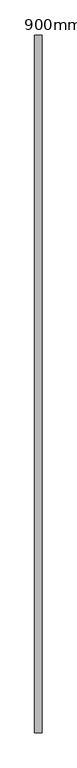
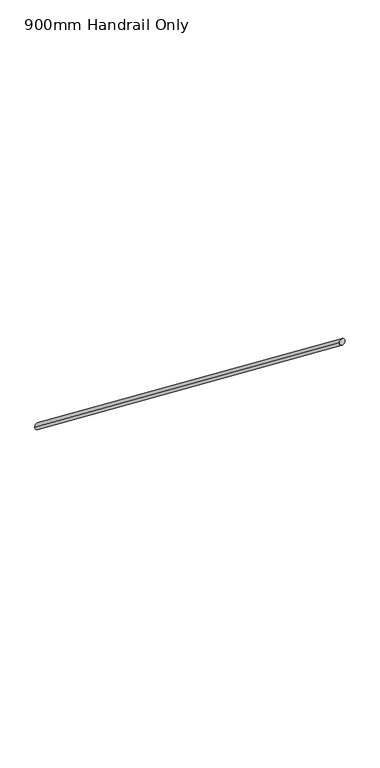
"""IFC4 building model written with IfcOpenShell, lengths in millimetres: railing geometry, 900mm Handrail Only."""

import ifcopenshell
import ifcopenshell.guid

model = None  # the IFC model being written
_history = None  # IfcOwnerHistory: only IFC2X3 demands one
_inside = {}  # id of a spatial element -> (the spatial element, [elements in it])
_under = {}  # id of a project, library or spatial element -> (it, [spatial elements below it])
_declared = {}  # id of a project -> (the project, [libraries it declares])
_typed = {}  # id of a type object -> (the type object, [elements of that type])
_made_of = {}  # id of a material, layer set ... -> (it, [elements and type objects made of it])


def new_model(schema):
    """Start an empty IFC model of exactly this schema.

    Asked for "IFC4X3", IfcOpenShell would pick the latest addendum, in which some entities
    have other attributes; the version numbers below select the first issue.
    IFC2X3 requires an IfcOwnerHistory on every rooted entity: one is made here for all.
    """
    global model, _history
    if schema == "IFC4X3":
        model = ifcopenshell.file(schema_version=(4, 3, 0, 0))
    else:
        model = ifcopenshell.file(schema=schema)
    _inside.clear()
    _under.clear()
    _declared.clear()
    _typed.clear()
    _made_of.clear()
    _history = None
    if model.schema == "IFC2X3":
        org = make("IfcOrganization", Name="unknown")
        user = make(
            "IfcPersonAndOrganization",
            ThePerson=make("IfcPerson", FamilyName="unknown"),
            TheOrganization=org,
        )
        app = make(
            "IfcApplication",
            ApplicationDeveloper=org,
            Version="unknown",
            ApplicationFullName="unknown",
            ApplicationIdentifier="unknown",
        )
        _history = make(
            "IfcOwnerHistory",
            OwningUser=user,
            OwningApplication=app,
            ChangeAction="ADDED",
            CreationDate=0,
        )
    return model


def make(cls, **values):
    """One entity of the class cls with the attributes given. An attribute that is None is left unset."""
    return model.create_entity(
        cls, **{name: value for name, value in values.items() if value is not None}
    )


def rooted(cls, **values):
    """An entity with a GlobalId (a new one), such as an element, a storey or a relation."""
    return make(cls, GlobalId=ifcopenshell.guid.new(), OwnerHistory=_history, **values)


def si_unit(unit_type, name, prefix=None):
    """IfcSIUnit, for example si_unit("LENGTHUNIT", "METRE", prefix="MILLI")."""
    return make("IfcSIUnit", UnitType=unit_type, Prefix=prefix, Name=name)


def assignment(units):
    """IfcUnitAssignment: the units of a project."""
    return None if units is None else make("IfcUnitAssignment", Units=units)


def point(xyz):
    """IfcCartesianPoint."""
    return None if xyz is None else make("IfcCartesianPoint", Coordinates=xyz)


def direction(xyz):
    """IfcDirection."""
    return None if xyz is None else make("IfcDirection", DirectionRatios=xyz)


def frame(location, z_axis=None, x_axis=None):
    """IfcAxis2Placement3D, a coordinate frame: its origin and axes. An axis left out is left unset."""
    return make(
        "IfcAxis2Placement3D",
        Location=point(location),
        Axis=direction(z_axis),
        RefDirection=direction(x_axis),
    )


def origin():
    """The frame at (0, 0, 0) with its axes left unset."""
    return frame((0.0, 0.0, 0.0))


def place(relative_to, where):
    """IfcLocalPlacement: puts the frame where relative to a parent placement (None: the world)."""
    return make(
        "IfcLocalPlacement", PlacementRelTo=relative_to, RelativePlacement=where
    )


def context(
    kind, dimensions, precision=None, world=None, true_north=None, identifier=None
):
    """IfcGeometricRepresentationContext, for example the 3D "Model" context."""
    return make(
        "IfcGeometricRepresentationContext",
        ContextIdentifier=identifier,
        ContextType=kind,
        CoordinateSpaceDimension=dimensions,
        Precision=precision,
        WorldCoordinateSystem=world,
        TrueNorth=true_north,
    )


def project(units=None, contexts=None):
    """IfcProject with its units and contexts."""
    return rooted(
        "IfcProject",
        Name="project",
        RepresentationContexts=contexts,
        UnitsInContext=assignment(units),
    )


def spatial(cls, under=None, at=None, **own):
    """A site, building, storey or space (cls), placed at a placement, below another one or the project."""
    s = rooted(cls, ObjectPlacement=at, **own)
    if under is not None:
        _under.setdefault(under.id(), (under, []))[1].append(s)
    return s


def ellipse_curve(where, semi_axis1, semi_axis2):
    """IfcEllipse in the frame where."""
    return make(
        "IfcEllipse", Position=where, SemiAxis1=semi_axis1, SemiAxis2=semi_axis2
    )


def shape(context_of_items, identifier, shape_type, items):
    """IfcShapeRepresentation: the items that make up one representation, for example the "Body"."""
    return make(
        "IfcShapeRepresentation",
        ContextOfItems=context_of_items,
        RepresentationIdentifier=identifier,
        RepresentationType=shape_type,
        Items=items,
    )


def source(mapping_origin, context_of_items, identifier, shape_type, items):
    """IfcRepresentationMap: a shape defined once, which mapped items show again and again."""
    return make(
        "IfcRepresentationMap",
        MappingOrigin=mapping_origin,
        MappedRepresentation=shape(context_of_items, identifier, shape_type, items),
    )


def transform(
    local_origin,
    x_axis=None,
    y_axis=None,
    z_axis=None,
    scale=None,
    scale2=None,
    scale3=None,
    uniform=True,
):
    """IfcCartesianTransformationOperator3D, or its non-uniform kind. x_axis, y_axis, z_axis: its Axis1, 2, 3."""
    if uniform:
        return make(
            "IfcCartesianTransformationOperator3D",
            Axis1=direction(x_axis),
            Axis2=direction(y_axis),
            LocalOrigin=point(local_origin),
            Scale=scale,
            Axis3=direction(z_axis),
        )
    return make(
        "IfcCartesianTransformationOperator3DnonUniform",
        Axis1=direction(x_axis),
        Axis2=direction(y_axis),
        LocalOrigin=point(local_origin),
        Scale=scale,
        Axis3=direction(z_axis),
        Scale2=scale2,
        Scale3=scale3,
    )


def mapped(mapping_source, mapping_target):
    """IfcMappedItem: shows the shape of a source again, moved by a transform."""
    return make(
        "IfcMappedItem", MappingSource=mapping_source, MappingTarget=mapping_target
    )


def made_of(thing, what):
    """Note that an element or type object is made of a material, layer set ...; save() writes the relation."""
    if what is not None:
        _made_of.setdefault(what.id(), (what, []))[1].append(thing)
    return thing


def element(
    cls,
    number,
    at=None,
    inside=None,
    cuts=None,
    type_object=None,
    material=None,
    context=None,
    identifier="Body",
    shape_type=None,
    held_by="IfcProductDefinitionShape",
    body=None,
    shapes=None,
    **own,
):
    """One element of the class cls, such as IfcWall. Its Tag is "e" and its number.

    at: its placement. inside: the storey or other place that contains it. cuts: it is an
    opening in that element (IfcRelVoidsElement). A single representation is given by context,
    identifier, shape_type and body (its items); several are given by shapes. held_by: the class
    of the entity that holds the representations. save() writes the other relations.
    """
    e = rooted(cls, Tag="e%d" % number, ObjectPlacement=at, **own)
    if body is not None:
        shapes = [shape(context, identifier, shape_type, body)]
    if shapes is not None:
        e.Representation = make(held_by, Representations=shapes)
    if inside is not None:
        _inside.setdefault(inside.id(), (inside, []))[1].append(e)
    if cuts is not None:
        rooted(
            "IfcRelVoidsElement", RelatingBuildingElement=cuts, RelatedOpeningElement=e
        )
    if type_object is not None:
        _typed.setdefault(type_object.id(), (type_object, []))[1].append(e)
    return made_of(e, material)


def aggregate(whole, parts):
    """IfcRelAggregates: a whole, such as a stair, and the parts it consists of."""
    return rooted("IfcRelAggregates", RelatingObject=whole, RelatedObjects=parts)


def save(model, path):
    """Write the relations noted so far, then the file.

    IfcRelAggregates (storeys below a building ...), IfcRelContainedInSpatialStructure (elements
    in a storey), IfcRelDefinesByType, IfcRelAssociatesMaterial and IfcRelDeclares: one each for
    every whole, place, type object, material and project.
    """
    for whole, parts in _under.values():
        aggregate(whole, parts)
    for where, things in _inside.values():
        rooted(
            "IfcRelContainedInSpatialStructure",
            RelatedElements=things,
            RelatingStructure=where,
        )
    for kind, things in _typed.values():
        rooted("IfcRelDefinesByType", RelatedObjects=things, RelatingType=kind)
    for what, things in _made_of.values():
        rooted("IfcRelAssociatesMaterial", RelatedObjects=things, RelatingMaterial=what)
    for by, libraries in _declared.values():
        rooted("IfcRelDeclares", RelatingContext=by, RelatedDefinitions=libraries)
    model.write(path)


def plane_surface(at):
    """IfcPlane: the flat surface through the origin of the frame at, square to its z axis."""
    return make("IfcPlane", Position=at)


def cylinder_surface(at, radius):
    """IfcCylindricalSurface: all points at the distance radius from the z axis of the frame at."""
    return make("IfcCylindricalSurface", Position=at, Radius=radius)


def advanced_brep(points, edges, surfaces, faces):
    """IfcAdvancedBrep: a solid bounded by faces that lie on surfaces and meet in shared edges.

    An edge is (start, end): straight between two places in points (the first is 0);
    or (start, end, curve); or (start, end, curve, False) where it runs against its curve.
    A face is (place in surfaces, loops), or (place, loops, False) where it looks against
    its surface's normal. A loop lists edges by number (the first is 1), with a minus sign
    where the edge is run from its end to its start. The first loop is the outer one.
    """
    corners = [point(p) for p in points]
    vertices = [make("IfcVertexPoint", VertexGeometry=c) for c in corners]
    made = []
    for start, end, *more in edges:
        made.append(
            make(
                "IfcEdgeCurve",
                EdgeStart=vertices[start],
                EdgeEnd=vertices[end],
                EdgeGeometry=more[0] if more else make("IfcPolyline", Points=[corners[start], corners[end]]),
                SameSense=more[1] if len(more) > 1 else True,
            )
        )
    hull = []
    for where, loops, *sense in faces:
        bounds = []
        for j, loop in enumerate(loops):
            ring = [make("IfcOrientedEdge", EdgeElement=made[abs(k) - 1], Orientation=k > 0) for k in loop]
            bounds.append(
                make(
                    "IfcFaceOuterBound" if j == 0 else "IfcFaceBound",
                    Bound=make("IfcEdgeLoop", EdgeList=ring),
                    Orientation=True,
                )
            )
        hull.append(make("IfcAdvancedFace", Bounds=bounds, FaceSurface=surfaces[where], SameSense=sense[0] if sense else True))
    return make("IfcAdvancedBrep", Outer=make("IfcClosedShell", CfsFaces=hull))


def railing_900mm_handrail_only_c6d3eaa9(model_context):
    return source(origin(), model_context, "Body", "AdvancedBrep", [
        advanced_brep(
        [(462.0, -5975.0, 1068.4468381), (422.0, -5975.0, 1068.4468381), (462.0, -9725.0, 3974.6968381), (422.0, -9725.0, 3974.6968381)],
        [
            (0, 1, ellipse_curve(frame((442.0, -5975.0, 1068.4468381), z_axis=(0.0, 1.0, 0.0), x_axis=(0.0, 0.0, -1.0)), 25.3031619, 20.0)),
            (1, 0, ellipse_curve(frame((442.0, -5975.0, 1068.4468381), z_axis=(0.0, 1.0, 0.0), x_axis=(0.0, 0.0, -1.0)), 25.3031619, 20.0)),
            (2, 3, ellipse_curve(frame((442.0, -9725.0, 3974.6968381), z_axis=(0.0, -1.0, 0.0), x_axis=(0.0, 0.0, -1.0)), 25.3031619, 20.0)),
            (3, 2, ellipse_curve(frame((442.0, -9725.0, 3974.6968381), z_axis=(0.0, -1.0, 0.0), x_axis=(0.0, 0.0, -1.0)), 25.3031619, 20.0)),
            (0, 2),
            (3, 1),
        ],
        [
            plane_surface(frame((442.0, -5975.0, 1093.75), z_axis=(0.0, 1.0, 0.0), x_axis=(0.0, 0.0, -1.0))),
            plane_surface(frame((442.0, -9725.0, 4000.0), z_axis=(0.0, -1.0, 0.0), x_axis=(0.0, 0.0, -1.0))),
            cylinder_surface(frame((442.0, -5987.2514333, 1077.941699), z_axis=(0.0, 0.7904150521752251, -0.612571665435838), x_axis=(-1.0, 0.0, 0.0)), 20.0),
        ],
        [
            (0, [[1, 2]]),
            (1, [[3, 4]]),
            (2, [[-1, 5, -4, 6]]),
            (2, [[-2, -6, -3, -5]]),
        ],
    ),
    ])


if __name__ == "__main__":
    model = new_model("IFC4")
    model_context = context("Model", 3, world=origin())
    ifc_project = project(units=[si_unit("LENGTHUNIT", "METRE", prefix="MILLI")], contexts=[model_context])
    site = spatial("IfcSite", under=ifc_project)
    building = spatial("IfcBuilding", under=site)
    placement = place(None, origin())
    railing_900mm_handrail_only_shape = railing_900mm_handrail_only_c6d3eaa9(model_context)
    element("IfcRailing", 1, ObjectType="900mm Handrail Only", at=placement, inside=building, context=model_context, shape_type="MappedRepresentation", body=[
        mapped(railing_900mm_handrail_only_shape, transform((0.0, 0.0, 0.0), x_axis=(1.0, 0.0, 0.0), y_axis=(0.0, 1.0, 0.0), z_axis=(0.0, 0.0, 1.0))),
    ])
    save(model, "model.ifc")
